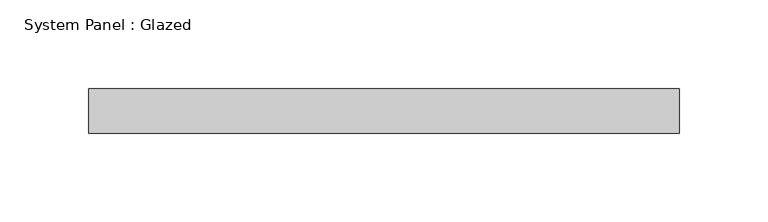
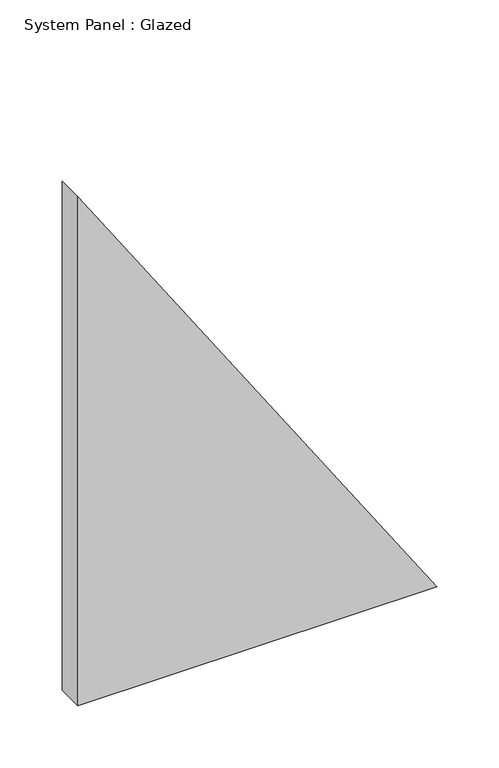
"""IFC4 building model written with IfcOpenShell, lengths in millimetres: plate geometry, System Panel : Glazed."""

from ifc_helpers import new_model, si_unit, frame, origin, place, context, project, spatial, polyline, outline, extrude, source, transform, mapped, element, save


def system_panel_glazed_5dcc9757(model_context):
    return source(origin(), model_context, "Body", "SweptSolid", [
        extrude(outline(polyline([(0.0, -166.474195), (0.0, 166.474195), (499.353934, -166.474195), (0.0, -166.474195)])), frame((0.0, 24.5, 0.0), z_axis=(0.0, 1.0, 0.0), x_axis=(0.0, 0.0, 1.0)), (0.0, 0.0, 1.0), 25.0),
    ])


if __name__ == "__main__":
    model = new_model("IFC4")
    model_context = context("Model", 3, world=origin())
    ifc_project = project(units=[si_unit("LENGTHUNIT", "METRE", prefix="MILLI")], contexts=[model_context])
    site = spatial("IfcSite", under=ifc_project)
    building = spatial("IfcBuilding", under=site)
    placement = place(None, origin())
    system_panel_glazed_shape = system_panel_glazed_5dcc9757(model_context)
    element("IfcPlate", 1, ObjectType="System Panel : Glazed", at=placement, inside=building, context=model_context, shape_type="MappedRepresentation", body=[
        mapped(system_panel_glazed_shape, transform((0.0, 0.0, 0.0), x_axis=(1.0, 0.0, 0.0), y_axis=(0.0, 1.0, 0.0), z_axis=(0.0, 0.0, 1.0))),
    ])
    save(model, "model.ifc")

# Revit data of these elements
# Type "System Panel : Glazed"
#   Keynote = "H11"
#   Construction Type Id = "GSP4R"
#   Analytic Construction = "1/8 in Pilkington single glazing"
#   Visual Light Transmittance = 0.9
#   Solar Heat Gain Coefficient = 0.86
#   Heat Transfer Coefficient (U) = 6.7069 W/(m²·K)
#   Define Thermal Properties by = 1
# Element 1 (IfcPlate, "System Panel : Glazed")
#   Materials on its faces: "Glass"
# Materials
#   "Glass": class "Glass", colour RGB 0 128 192, transparency 0.9, Description = "Soda Lime Glass", Cost = 0
